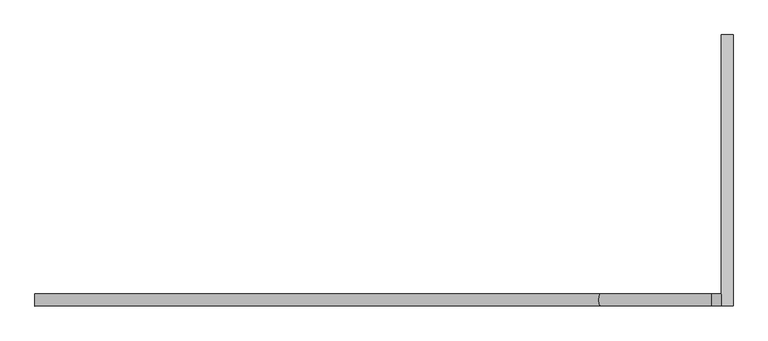
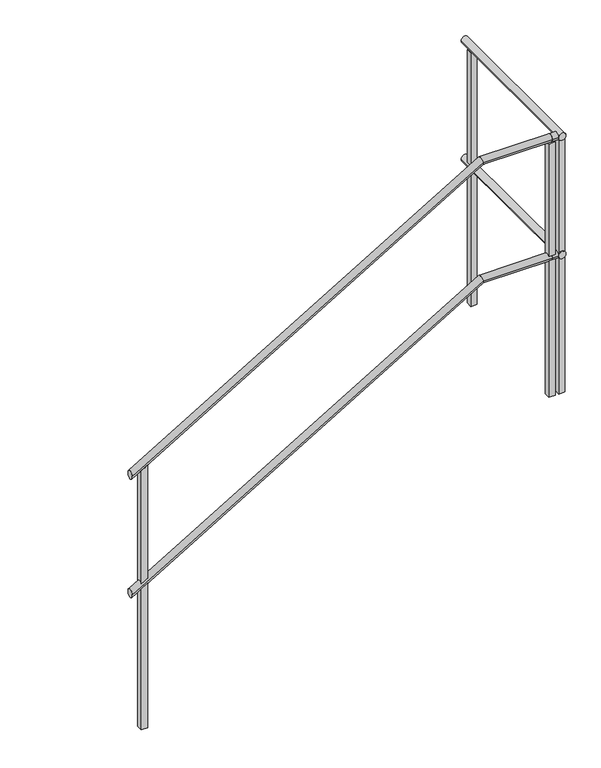
"""IFC4 building model written with IfcOpenShell, lengths in millimetres: railing geometry."""

from ifc_helpers import new_model, si_unit, frame, origin, place, context, project, spatial, polyline, circle_curve, ellipse_curve, outline, extrude, source, transform, mapped, element, save
from ifc_brep_helpers import plane_surface, cylinder_surface, advanced_brep


def railing_007d1d3f(model_context):
    return source(origin(), model_context, "Body", "SolidModel", [
        advanced_brep(
        [(35195.0, 4.9208589, 899.1723166), (35195.0, -25.0791411, 899.1723166), (36599.1264386, 4.9208589, 1734.9618634), (36599.1264386, -25.0791411, 1734.9618634), (36875.0, 4.9208589, 1734.9618634), (36875.0, -25.0791411, 1734.9618634)],
        [
            (0, 1, ellipse_curve(frame((35195.0, -10.0791411, 899.1723166), z_axis=(-1.0, 0.0, 0.0), x_axis=(0.0, 0.0, -1.0)), 17.4562134, 15.0)),
            (1, 0, ellipse_curve(frame((35195.0, -10.0791411, 899.1723166), z_axis=(-1.0, 0.0, 0.0), x_axis=(0.0, 0.0, -1.0)), 17.4562134, 15.0)),
            (0, 2),
            (2, 3, ellipse_curve(frame((36599.1264386, -10.0791411, 1734.9618634), z_axis=(-0.9641817474962143, 0.0, -0.265242450967311), x_axis=(0.265242450967311, 0.0, -0.9641817474962145)), 15.5572329, 15.0)),
            (3, 1),
            (3, 2, ellipse_curve(frame((36599.1264386, -10.0791411, 1734.9618634), z_axis=(-0.9641817474962143, 0.0, -0.265242450967311), x_axis=(0.265242450967311, 0.0, -0.9641817474962145)), 15.5572329, 15.0)),
            (4, 5, circle_curve(frame((36875.0, -10.0791411, 1734.9618634), z_axis=(1.0, 0.0, 0.0), x_axis=(0.0, -1.0, 0.0)), 15.0)),
            (5, 4, circle_curve(frame((36875.0, -10.0791411, 1734.9618634), z_axis=(1.0, 0.0, 0.0), x_axis=(0.0, -1.0, 0.0)), 15.0)),
            (2, 4),
            (5, 3),
        ],
        [
            plane_surface(frame((35195.0, -10.0791411, 916.62853), z_axis=(-1.0, 0.0, 0.0), x_axis=(0.0, 1.0, 0.0))),
            cylinder_surface(frame((35202.6722579, -10.0791411, 903.7391368), z_axis=(-0.8592928844097072, 0.0, -0.5114838597676818), x_axis=(0.0, -1.0, 0.0)), 15.0),
            plane_surface(frame((36875.0, -10.0791411, 1749.9618634), z_axis=(1.0, 0.0, 0.0), x_axis=(0.0, 1.0, 0.0))),
            cylinder_surface(frame((36595.0, -10.0791411, 1734.9618634), z_axis=(-1.0, 0.0, 0.0), x_axis=(0.0, -1.0, 0.0)), 15.0),
        ],
        [
            (0, [[1, 2]]),
            (1, [[-1, 3, 4, 5]]),
            (1, [[-2, -5, 6, -3]]),
            (2, [[7, 8]]),
            (3, [[-4, 9, -8, 10]]),
            (3, [[-6, -10, -7, -9]]),
        ],
    ),
        advanced_brep(
        [(36875.0, 4.9208589, 1734.9618634), (36875.0, -25.0791411, 1734.9618634), (36899.6, 4.9208589, 1734.9618634), (36899.6, -25.0791411, 1734.9618634)],
        [
            (0, 1, circle_curve(frame((36875.0, -10.0791411, 1734.9618634), z_axis=(-1.0, 0.0, 0.0), x_axis=(0.0, -1.0, 0.0)), 15.0)),
            (1, 0, circle_curve(frame((36875.0, -10.0791411, 1734.9618634), z_axis=(-1.0, 0.0, 0.0), x_axis=(0.0, -1.0, 0.0)), 15.0)),
            (2, 3, circle_curve(frame((36899.6, -10.0791411, 1734.9618634), z_axis=(1.0, 0.0, 0.0), x_axis=(0.0, -1.0, 0.0)), 15.0)),
            (3, 2, circle_curve(frame((36899.6, -10.0791411, 1734.9618634), z_axis=(1.0, 0.0, 0.0), x_axis=(0.0, -1.0, 0.0)), 15.0)),
            (0, 2),
            (3, 1),
        ],
        [
            plane_surface(frame((36875.0, -10.0791411, 1749.9618634), z_axis=(-1.0, 0.0, 0.0), x_axis=(0.0, 1.0, 0.0))),
            plane_surface(frame((36899.6, -10.0791411, 1749.9618634), z_axis=(1.0, 0.0, 0.0), x_axis=(0.0, 1.0, 0.0))),
            cylinder_surface(frame((36875.0, -10.0791411, 1734.9618634), z_axis=(-1.0, 0.0, 0.0), x_axis=(0.0, -1.0, 0.0)), 15.0),
        ],
        [
            (0, [[1, 2]]),
            (1, [[3, 4]]),
            (2, [[-1, 5, -4, 6]]),
            (2, [[-2, -6, -3, -5]]),
        ],
    ),
        advanced_brep(
        [(36899.6, -25.0791411, 1734.9618634), (36929.6, -25.0791411, 1734.9618634), (36899.6, 649.5208589, 1734.9618634), (36929.6, 649.5208589, 1734.9618634)],
        [
            (0, 1, circle_curve(frame((36914.6, -25.0791411, 1734.9618634), z_axis=(0.0, -1.0, 0.0), x_axis=(1.0, 0.0, 0.0)), 15.0)),
            (1, 0, circle_curve(frame((36914.6, -25.0791411, 1734.9618634), z_axis=(0.0, -1.0, 0.0), x_axis=(1.0, 0.0, 0.0)), 15.0)),
            (2, 3, circle_curve(frame((36914.6, 649.5208589, 1734.9618634), z_axis=(0.0, 1.0, 0.0), x_axis=(1.0, 0.0, 0.0)), 15.0)),
            (3, 2, circle_curve(frame((36914.6, 649.5208589, 1734.9618634), z_axis=(0.0, 1.0, 0.0), x_axis=(1.0, 0.0, 0.0)), 15.0)),
            (0, 2),
            (3, 1),
        ],
        [
            plane_surface(frame((36914.6, -25.0791411, 1749.9618634), z_axis=(0.0, -1.0, 0.0), x_axis=(0.0, 0.0, 1.0))),
            plane_surface(frame((36914.6, 649.5208589, 1749.9618634), z_axis=(0.0, 1.0, 0.0), x_axis=(0.0, 0.0, 1.0))),
            cylinder_surface(frame((36914.6, -25.0791411, 1734.9618634), z_axis=(0.0, -1.0, 0.0), x_axis=(1.0, 0.0, 0.0)), 15.0),
        ],
        [
            (0, [[1, 2]]),
            (1, [[3, 4]]),
            (2, [[-1, 5, -4, 6]]),
            (2, [[-2, -6, -3, -5]]),
        ],
    ),
        advanced_brep(
        [(35195.0, 4.9208589, 1399.1723166), (35195.0, -25.0791411, 1399.1723166), (36599.1264386, 4.9208589, 2234.9618634), (36599.1264386, -25.0791411, 2234.9618634), (36875.0, 4.9208589, 2234.9618634), (36875.0, -25.0791411, 2234.9618634)],
        [
            (0, 1, ellipse_curve(frame((35195.0, -10.0791411, 1399.1723166), z_axis=(-1.0, 0.0, 0.0), x_axis=(0.0, 0.0, -1.0)), 17.4562134, 15.0)),
            (1, 0, ellipse_curve(frame((35195.0, -10.0791411, 1399.1723166), z_axis=(-1.0, 0.0, 0.0), x_axis=(0.0, 0.0, -1.0)), 17.4562134, 15.0)),
            (0, 2),
            (2, 3, ellipse_curve(frame((36599.1264386, -10.0791411, 2234.9618634), z_axis=(-0.9641817474962143, 0.0, -0.265242450967311), x_axis=(0.265242450967311, 0.0, -0.9641817474962145)), 15.5572329, 15.0)),
            (3, 1),
            (3, 2, ellipse_curve(frame((36599.1264386, -10.0791411, 2234.9618634), z_axis=(-0.9641817474962143, 0.0, -0.265242450967311), x_axis=(0.265242450967311, 0.0, -0.9641817474962145)), 15.5572329, 15.0)),
            (4, 5, circle_curve(frame((36875.0, -10.0791411, 2234.9618634), z_axis=(1.0, 0.0, 0.0), x_axis=(0.0, -1.0, 0.0)), 15.0)),
            (5, 4, circle_curve(frame((36875.0, -10.0791411, 2234.9618634), z_axis=(1.0, 0.0, 0.0), x_axis=(0.0, -1.0, 0.0)), 15.0)),
            (2, 4),
            (5, 3),
        ],
        [
            plane_surface(frame((35195.0, -10.0791411, 1416.62853), z_axis=(-1.0, 0.0, 0.0), x_axis=(0.0, 1.0, 0.0))),
            cylinder_surface(frame((35202.6722579, -10.0791411, 1403.7391368), z_axis=(-0.8592928844097072, 0.0, -0.5114838597676818), x_axis=(0.0, -1.0, 0.0)), 15.0),
            plane_surface(frame((36875.0, -10.0791411, 2249.9618634), z_axis=(1.0, 0.0, 0.0), x_axis=(0.0, 1.0, 0.0))),
            cylinder_surface(frame((36595.0, -10.0791411, 2234.9618634), z_axis=(-1.0, 0.0, 0.0), x_axis=(0.0, -1.0, 0.0)), 15.0),
        ],
        [
            (0, [[1, 2]]),
            (1, [[-1, 3, 4, 5]]),
            (1, [[-2, -5, 6, -3]]),
            (2, [[7, 8]]),
            (3, [[-4, 9, -8, 10]]),
            (3, [[-6, -10, -7, -9]]),
        ],
    ),
        advanced_brep(
        [(36875.0, 4.9208589, 2234.9618634), (36875.0, -25.0791411, 2234.9618634), (36899.6, 4.9208589, 2234.9618634), (36899.6, -25.0791411, 2234.9618634)],
        [
            (0, 1, circle_curve(frame((36875.0, -10.0791411, 2234.9618634), z_axis=(-1.0, 0.0, 0.0), x_axis=(0.0, -1.0, 0.0)), 15.0)),
            (1, 0, circle_curve(frame((36875.0, -10.0791411, 2234.9618634), z_axis=(-1.0, 0.0, 0.0), x_axis=(0.0, -1.0, 0.0)), 15.0)),
            (2, 3, circle_curve(frame((36899.6, -10.0791411, 2234.9618634), z_axis=(1.0, 0.0, 0.0), x_axis=(0.0, -1.0, 0.0)), 15.0)),
            (3, 2, circle_curve(frame((36899.6, -10.0791411, 2234.9618634), z_axis=(1.0, 0.0, 0.0), x_axis=(0.0, -1.0, 0.0)), 15.0)),
            (0, 2),
            (3, 1),
        ],
        [
            plane_surface(frame((36875.0, -10.0791411, 2249.9618634), z_axis=(-1.0, 0.0, 0.0), x_axis=(0.0, 1.0, 0.0))),
            plane_surface(frame((36899.6, -10.0791411, 2249.9618634), z_axis=(1.0, 0.0, 0.0), x_axis=(0.0, 1.0, 0.0))),
            cylinder_surface(frame((36875.0, -10.0791411, 2234.9618634), z_axis=(-1.0, 0.0, 0.0), x_axis=(0.0, -1.0, 0.0)), 15.0),
        ],
        [
            (0, [[1, 2]]),
            (1, [[3, 4]]),
            (2, [[-1, 5, -4, 6]]),
            (2, [[-2, -6, -3, -5]]),
        ],
    ),
        advanced_brep(
        [(36899.6, -25.0791411, 2234.9618634), (36929.6, -25.0791411, 2234.9618634), (36899.6, 649.5208589, 2234.9618634), (36929.6, 649.5208589, 2234.9618634)],
        [
            (0, 1, circle_curve(frame((36914.6, -25.0791411, 2234.9618634), z_axis=(0.0, -1.0, 0.0), x_axis=(1.0, 0.0, 0.0)), 15.0)),
            (1, 0, circle_curve(frame((36914.6, -25.0791411, 2234.9618634), z_axis=(0.0, -1.0, 0.0), x_axis=(1.0, 0.0, 0.0)), 15.0)),
            (2, 3, circle_curve(frame((36914.6, 649.5208589, 2234.9618634), z_axis=(0.0, 1.0, 0.0), x_axis=(1.0, 0.0, 0.0)), 15.0)),
            (3, 2, circle_curve(frame((36914.6, 649.5208589, 2234.9618634), z_axis=(0.0, 1.0, 0.0), x_axis=(1.0, 0.0, 0.0)), 15.0)),
            (0, 2),
            (3, 1),
        ],
        [
            plane_surface(frame((36914.6, -25.0791411, 2249.9618634), z_axis=(0.0, -1.0, 0.0), x_axis=(0.0, 0.0, 1.0))),
            plane_surface(frame((36914.6, 649.5208589, 2249.9618634), z_axis=(0.0, 1.0, 0.0), x_axis=(0.0, 0.0, 1.0))),
            cylinder_surface(frame((36914.6, -25.0791411, 2234.9618634), z_axis=(0.0, -1.0, 0.0), x_axis=(1.0, 0.0, 0.0)), 15.0),
        ],
        [
            (0, [[1, 2]]),
            (1, [[3, 4]]),
            (2, [[-1, 5, -4, 6]]),
            (2, [[-2, -6, -3, -5]]),
        ],
    ),
        extrude(outline(polyline([(36902.1, -22.5791411), (36902.1, 2.4208589), (36927.1, 2.4208589), (36927.1, -22.5791411), (36902.1, -22.5791411)])), frame((0.0, 0.0, 1149.9618634), z_axis=(0.0, 0.0, 1.0), x_axis=(1.0, 0.0, 0.0)), (0.0, 0.0, 1.0), 1070.0),
        extrude(outline(polyline([(36862.5, -22.5791411), (36862.5, 2.4208589), (36887.5, 2.4208589), (36887.5, -22.5791411), (36862.5, -22.5791411)])), frame((0.0, 0.0, 1149.9618634), z_axis=(0.0, 0.0, 1.0), x_axis=(1.0, 0.0, 0.0)), (0.0, 0.0, 1.0), 1070.0),
        extrude(outline(polyline([(36927.1, 587.0208589), (36902.1, 587.0208589), (36902.1, 612.0208589), (36927.1, 612.0208589), (36927.1, 587.0208589)])), frame((0.0, 0.0, 1149.9618634), z_axis=(0.0, 0.0, 1.0), x_axis=(1.0, 0.0, 0.0)), (0.0, 0.0, 1.0), 1070.0),
        extrude(outline(polyline([(1408.9499586, 35232.5), (316.62853, 35232.5), (316.62853, 35257.5), (1423.830911, 35257.5), (1408.9499586, 35232.5)])), frame((0.0, -22.5791411, 0.0), z_axis=(0.0, 1.0, 0.0), x_axis=(0.0, 0.0, 1.0)), (0.0, 0.0, 1.0), 25.0),
    ])


if __name__ == "__main__":
    model = new_model("IFC4")
    model_context = context("Model", 3, world=origin())
    ifc_project = project(units=[si_unit("LENGTHUNIT", "METRE", prefix="MILLI")], contexts=[model_context])
    site = spatial("IfcSite", under=ifc_project)
    building = spatial("IfcBuilding", under=site)
    placement = place(None, origin())
    railing_shape = railing_007d1d3f(model_context)
    element("IfcRailing", 1, at=placement, inside=building, context=model_context, shape_type="MappedRepresentation", body=[
        mapped(railing_shape, transform((0.0, 0.0, 0.0), x_axis=(1.0, 0.0, 0.0), y_axis=(0.0, 1.0, 0.0), z_axis=(0.0, 0.0, 1.0))),
    ])
    save(model, "model.ifc")
